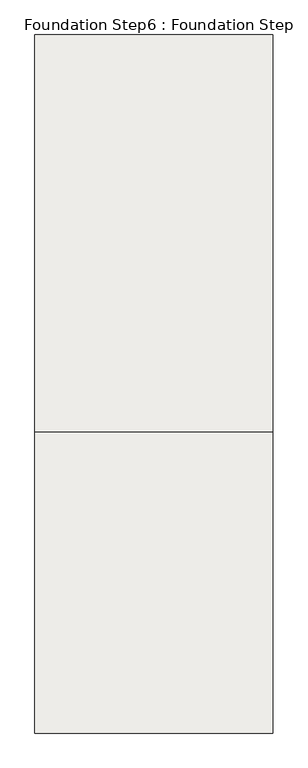
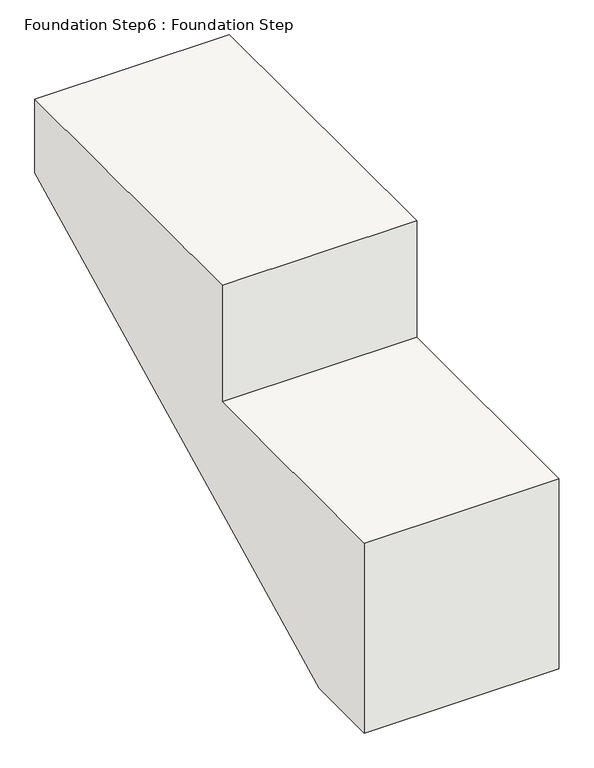
"""IFC4 building model written with IfcOpenShell, lengths in millimetres: slab geometry, Foundation Step6 : Foundation Step."""

from ifc_helpers import new_model, si_unit, frame, origin, place, context, project, spatial, polyline, outline, extrude, source, transform, mapped, element, save


def foundation_step6_foundation_step_ef98733d(model_context):
    return source(origin(), model_context, "Body", "SweptSolid", [
        extrude(outline(polyline([(-9123.6231529, -2362.2), (-9123.6231529, -1574.8), (-8158.4231529, -1574.8), (-8158.4231529, -1092.2), (-6888.4231529, -1092.2), (-6888.4231529, -1397.0), (-8818.8231529, -2362.2), (-9123.6231529, -2362.2)])), frame((-49611.0100821, 0.0, 0.0), z_axis=(1.0, 0.0, 0.0), x_axis=(0.0, 1.0, 0.0)), (0.0, 0.0, 1.0), 762.0),
    ])


if __name__ == "__main__":
    model = new_model("IFC4")
    model_context = context("Model", 3, world=origin())
    ifc_project = project(units=[si_unit("LENGTHUNIT", "METRE", prefix="MILLI")], contexts=[model_context])
    site = spatial("IfcSite", under=ifc_project)
    building = spatial("IfcBuilding", under=site)
    placement = place(None, origin())
    foundation_step6_foundation_step_shape = foundation_step6_foundation_step_ef98733d(model_context)
    element("IfcSlab", 1, ObjectType="Foundation Step6 : Foundation Step", at=placement, inside=building, context=model_context, shape_type="MappedRepresentation", body=[
        mapped(foundation_step6_foundation_step_shape, transform((0.0, 0.0, 0.0), x_axis=(1.0, 0.0, 0.0), y_axis=(0.0, 1.0, 0.0), z_axis=(0.0, 0.0, 1.0))),
    ])
    save(model, "model.ifc")

# Revit data of these elements
# Type "Foundation Step6 : Foundation Step"
#   Structural Material = Concrete, Cast-in-Place gray
# Materials
#   "Concrete, Cast-in-Place gray": class "Concrete", colour RGB 192 192 192, transparency 0, Description = "Cast-in-place concrete", Cost = 0
